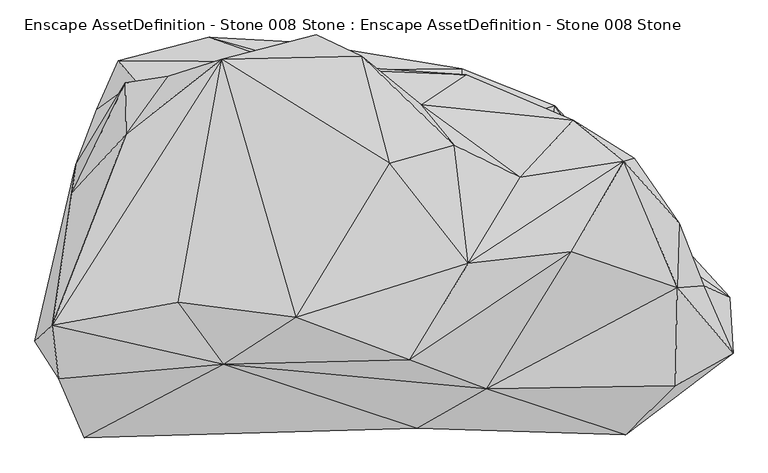
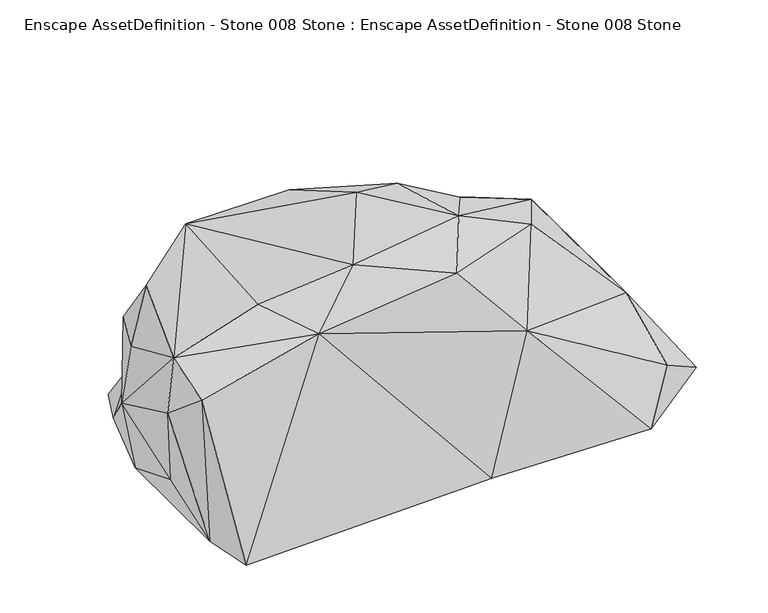
"""IFC4 building model written with IfcOpenShell, lengths in millimetres: geographic element geometry, Enscape AssetDefinition - Stone 008 Stone : Enscape AssetDefinition - Stone 008 Stone."""

import ifcopenshell
import ifcopenshell.guid

model = None  # the IFC model being written
_history = None  # IfcOwnerHistory: only IFC2X3 demands one
_inside = {}  # id of a spatial element -> (the spatial element, [elements in it])
_under = {}  # id of a project, library or spatial element -> (it, [spatial elements below it])
_declared = {}  # id of a project -> (the project, [libraries it declares])
_typed = {}  # id of a type object -> (the type object, [elements of that type])
_made_of = {}  # id of a material, layer set ... -> (it, [elements and type objects made of it])


def new_model(schema):
    """Start an empty IFC model of exactly this schema.

    Asked for "IFC4X3", IfcOpenShell would pick the latest addendum, in which some entities
    have other attributes; the version numbers below select the first issue.
    IFC2X3 requires an IfcOwnerHistory on every rooted entity: one is made here for all.
    """
    global model, _history
    if schema == "IFC4X3":
        model = ifcopenshell.file(schema_version=(4, 3, 0, 0))
    else:
        model = ifcopenshell.file(schema=schema)
    _inside.clear()
    _under.clear()
    _declared.clear()
    _typed.clear()
    _made_of.clear()
    _history = None
    if model.schema == "IFC2X3":
        org = make("IfcOrganization", Name="unknown")
        user = make(
            "IfcPersonAndOrganization",
            ThePerson=make("IfcPerson", FamilyName="unknown"),
            TheOrganization=org,
        )
        app = make(
            "IfcApplication",
            ApplicationDeveloper=org,
            Version="unknown",
            ApplicationFullName="unknown",
            ApplicationIdentifier="unknown",
        )
        _history = make(
            "IfcOwnerHistory",
            OwningUser=user,
            OwningApplication=app,
            ChangeAction="ADDED",
            CreationDate=0,
        )
    return model


def make(cls, **values):
    """One entity of the class cls with the attributes given. An attribute that is None is left unset."""
    return model.create_entity(
        cls, **{name: value for name, value in values.items() if value is not None}
    )


def rooted(cls, **values):
    """An entity with a GlobalId (a new one), such as an element, a storey or a relation."""
    return make(cls, GlobalId=ifcopenshell.guid.new(), OwnerHistory=_history, **values)


def si_unit(unit_type, name, prefix=None):
    """IfcSIUnit, for example si_unit("LENGTHUNIT", "METRE", prefix="MILLI")."""
    return make("IfcSIUnit", UnitType=unit_type, Prefix=prefix, Name=name)


def assignment(units):
    """IfcUnitAssignment: the units of a project."""
    return None if units is None else make("IfcUnitAssignment", Units=units)


def point(xyz):
    """IfcCartesianPoint."""
    return None if xyz is None else make("IfcCartesianPoint", Coordinates=xyz)


def direction(xyz):
    """IfcDirection."""
    return None if xyz is None else make("IfcDirection", DirectionRatios=xyz)


def frame(location, z_axis=None, x_axis=None):
    """IfcAxis2Placement3D, a coordinate frame: its origin and axes. An axis left out is left unset."""
    return make(
        "IfcAxis2Placement3D",
        Location=point(location),
        Axis=direction(z_axis),
        RefDirection=direction(x_axis),
    )


def origin():
    """The frame at (0, 0, 0) with its axes left unset."""
    return frame((0.0, 0.0, 0.0))


def place(relative_to, where):
    """IfcLocalPlacement: puts the frame where relative to a parent placement (None: the world)."""
    return make(
        "IfcLocalPlacement", PlacementRelTo=relative_to, RelativePlacement=where
    )


def context(
    kind, dimensions, precision=None, world=None, true_north=None, identifier=None
):
    """IfcGeometricRepresentationContext, for example the 3D "Model" context."""
    return make(
        "IfcGeometricRepresentationContext",
        ContextIdentifier=identifier,
        ContextType=kind,
        CoordinateSpaceDimension=dimensions,
        Precision=precision,
        WorldCoordinateSystem=world,
        TrueNorth=true_north,
    )


def project(units=None, contexts=None):
    """IfcProject with its units and contexts."""
    return rooted(
        "IfcProject",
        Name="project",
        RepresentationContexts=contexts,
        UnitsInContext=assignment(units),
    )


def spatial(cls, under=None, at=None, **own):
    """A site, building, storey or space (cls), placed at a placement, below another one or the project."""
    s = rooted(cls, ObjectPlacement=at, **own)
    if under is not None:
        _under.setdefault(under.id(), (under, []))[1].append(s)
    return s


def faces_of(points, faces, orient=None, outer=None):
    """IfcFace entities. A face is a list of loops; a loop is a list of indices into points, from 0.

    orient and outer hold one flag for each loop. By default every Orientation is true, the
    first loop of a face is its IfcFaceOuterBound and the others are IfcFaceBound.
    """
    made = []
    for i, loops in enumerate(faces):
        bounds = []
        for j, loop in enumerate(loops):
            is_outer = j == 0 if outer is None else outer[i][j]
            bounds.append(
                make(
                    "IfcFaceOuterBound" if is_outer else "IfcFaceBound",
                    Bound=make("IfcPolyLoop", Polygon=[points[k] for k in loop]),
                    Orientation=True if orient is None else orient[i][j],
                )
            )
        made.append(make("IfcFace", Bounds=bounds))
    return made


def faceted_brep(points, faces, orient=None, outer=None, voids=None):
    """IfcFacetedBrep: a solid bounded by flat faces; with voids (closed shells), ...WithVoids."""
    shared = [point(p) for p in points]
    hull = make("IfcClosedShell", CfsFaces=faces_of(shared, faces, orient, outer))
    if voids is None:
        return make("IfcFacetedBrep", Outer=hull)
    return make(
        "IfcFacetedBrepWithVoids",
        Outer=hull,
        Voids=[
            make(cls, CfsFaces=faces_of(shared, fs, o, b)) for cls, fs, o, b in voids
        ],
    )


def shape(context_of_items, identifier, shape_type, items):
    """IfcShapeRepresentation: the items that make up one representation, for example the "Body"."""
    return make(
        "IfcShapeRepresentation",
        ContextOfItems=context_of_items,
        RepresentationIdentifier=identifier,
        RepresentationType=shape_type,
        Items=items,
    )


def source(mapping_origin, context_of_items, identifier, shape_type, items):
    """IfcRepresentationMap: a shape defined once, which mapped items show again and again."""
    return make(
        "IfcRepresentationMap",
        MappingOrigin=mapping_origin,
        MappedRepresentation=shape(context_of_items, identifier, shape_type, items),
    )


def transform(
    local_origin,
    x_axis=None,
    y_axis=None,
    z_axis=None,
    scale=None,
    scale2=None,
    scale3=None,
    uniform=True,
):
    """IfcCartesianTransformationOperator3D, or its non-uniform kind. x_axis, y_axis, z_axis: its Axis1, 2, 3."""
    if uniform:
        return make(
            "IfcCartesianTransformationOperator3D",
            Axis1=direction(x_axis),
            Axis2=direction(y_axis),
            LocalOrigin=point(local_origin),
            Scale=scale,
            Axis3=direction(z_axis),
        )
    return make(
        "IfcCartesianTransformationOperator3DnonUniform",
        Axis1=direction(x_axis),
        Axis2=direction(y_axis),
        LocalOrigin=point(local_origin),
        Scale=scale,
        Axis3=direction(z_axis),
        Scale2=scale2,
        Scale3=scale3,
    )


def mapped(mapping_source, mapping_target):
    """IfcMappedItem: shows the shape of a source again, moved by a transform."""
    return make(
        "IfcMappedItem", MappingSource=mapping_source, MappingTarget=mapping_target
    )


def made_of(thing, what):
    """Note that an element or type object is made of a material, layer set ...; save() writes the relation."""
    if what is not None:
        _made_of.setdefault(what.id(), (what, []))[1].append(thing)
    return thing


def element(
    cls,
    number,
    at=None,
    inside=None,
    cuts=None,
    type_object=None,
    material=None,
    context=None,
    identifier="Body",
    shape_type=None,
    held_by="IfcProductDefinitionShape",
    body=None,
    shapes=None,
    **own,
):
    """One element of the class cls, such as IfcWall. Its Tag is "e" and its number.

    at: its placement. inside: the storey or other place that contains it. cuts: it is an
    opening in that element (IfcRelVoidsElement). A single representation is given by context,
    identifier, shape_type and body (its items); several are given by shapes. held_by: the class
    of the entity that holds the representations. save() writes the other relations.
    """
    e = rooted(cls, Tag="e%d" % number, ObjectPlacement=at, **own)
    if body is not None:
        shapes = [shape(context, identifier, shape_type, body)]
    if shapes is not None:
        e.Representation = make(held_by, Representations=shapes)
    if inside is not None:
        _inside.setdefault(inside.id(), (inside, []))[1].append(e)
    if cuts is not None:
        rooted(
            "IfcRelVoidsElement", RelatingBuildingElement=cuts, RelatedOpeningElement=e
        )
    if type_object is not None:
        _typed.setdefault(type_object.id(), (type_object, []))[1].append(e)
    return made_of(e, material)


def aggregate(whole, parts):
    """IfcRelAggregates: a whole, such as a stair, and the parts it consists of."""
    return rooted("IfcRelAggregates", RelatingObject=whole, RelatedObjects=parts)


def save(model, path):
    """Write the relations noted so far, then the file.

    IfcRelAggregates (storeys below a building ...), IfcRelContainedInSpatialStructure (elements
    in a storey), IfcRelDefinesByType, IfcRelAssociatesMaterial and IfcRelDeclares: one each for
    every whole, place, type object, material and project.
    """
    for whole, parts in _under.values():
        aggregate(whole, parts)
    for where, things in _inside.values():
        rooted(
            "IfcRelContainedInSpatialStructure",
            RelatedElements=things,
            RelatingStructure=where,
        )
    for kind, things in _typed.values():
        rooted("IfcRelDefinesByType", RelatedObjects=things, RelatingType=kind)
    for what, things in _made_of.values():
        rooted("IfcRelAssociatesMaterial", RelatedObjects=things, RelatingMaterial=what)
    for by, libraries in _declared.values():
        rooted("IfcRelDeclares", RelatingContext=by, RelatedDefinitions=libraries)
    model.write(path)


def enscape_assetdefinition_stone_008_stone_enscape_24533d0f(model_context):
    return source(origin(), model_context, "Body", "Brep", [
        faceted_brep([(674.4772792, 188.1209314, 142.7758336), (1035.7327461, 8.9201359, 108.4343269), (705.4293752, 497.0492125, 9.8005356), (997.1603155, 302.5434315, 403.4194052), (1162.8789902, 63.3667782, 307.4120581), (1253.1027794, -166.4617509, 132.1936697), (1349.0210772, -208.1131637, 6.9734799), (358.8430882, 390.0140226, 146.3160366), (377.8702021, 610.8905673, 436.6148412), (958.5034251, 293.037504, 588.9674425), (772.0807195, 443.9393878, 571.6524124), (1155.1955938, -174.3785888, 316.583544), (1361.7579937, -414.6891236, 4.4628736), (966.4069414, -714.6763802, 5.4843184), (1148.0065584, -535.101831, 161.3812745), (454.9190998, -545.4375148, 589.6245837), (765.6313181, -41.1196649, 728.256464), (197.4091679, -690.6881928, 2.2398918), (-514.082849, -456.0222328, 858.2776785), (170.5874205, -438.8919473, 922.1434593), (385.2636814, -83.5196525, 931.4427376), (-247.4171519, -282.6159894, 1018.4793472), (576.8572688, 233.5522175, 768.9470053), (335.1638615, 351.0840833, 853.2254696), (97.4461734, 284.5808566, 931.3715696), (213.0276859, 499.7121692, 607.2036028), (-6.4782458, 678.3997416, 740.2927279), (-523.0283737, 667.5286889, 753.1849146), (-682.7530861, -228.3637375, 932.9548478), (-874.7516274, 392.5074339, 724.0793109), (-1147.2679377, -313.0920827, 869.5514202), (-173.4227836, 757.5678229, 583.3979845), (-719.4939852, 606.0778499, 573.5012889), (-121.4118823, 631.9727302, 438.7468398), (-477.7078629, 640.0285363, 443.1231916), (-877.9751062, 580.4912448, 445.3162253), (-1074.303627, 173.3499914, 609.6158624), (-1061.0442162, 279.8386514, 242.5745577), (-839.9647474, 586.9014859, 173.4158546), (-312.4943078, 658.5144997, 220.8529711), (-903.9554596, 662.9179716, 4.3747872), (-983.217001, 483.1243753, 17.7407339), (-570.9864497, 749.253273, 0.3116064), (-136.2574697, 627.3009181, 146.1777389), (-233.8543534, 731.0650349, 7.1665621), (362.7277911, 632.3495507, 5.9714052), (-1086.7136717, 120.3676835, 13.3715561), (-1058.6297512, -132.5317025, 94.683297), (-1091.7432308, -525.1657367, 26.3983011), (-1029.1792154, -726.3221741, 1.9205989), (-1210.739255, -371.0243106, 639.5069957), (-1122.2990751, -508.4093809, 759.0334415)], [[[0, 1, 2]], [[3, 4, 1]], [[4, 5, 1]], [[1, 5, 6]], [[3, 1, 0]], [[2, 1, 6]], [[0, 2, 7]], [[7, 8, 0]], [[0, 8, 3]], [[3, 9, 4]], [[10, 3, 8]], [[3, 10, 9]], [[9, 11, 4]], [[4, 11, 5]], [[12, 5, 11]], [[12, 6, 5]], [[13, 2, 6]], [[13, 6, 12]], [[12, 11, 14]], [[12, 14, 13]], [[11, 15, 14]], [[16, 15, 11]], [[11, 9, 16]], [[14, 15, 13]], [[13, 15, 17]], [[13, 17, 2]], [[18, 15, 19]], [[16, 19, 15]], [[18, 17, 15]], [[16, 20, 19]], [[16, 9, 20]], [[21, 19, 20]], [[21, 18, 19]], [[9, 22, 20]], [[20, 22, 23]], [[20, 23, 24]], [[24, 21, 20]], [[10, 22, 9]], [[23, 22, 25]], [[25, 22, 10]], [[23, 26, 24]], [[25, 26, 23]], [[27, 21, 24]], [[27, 24, 26]], [[27, 28, 21]], [[18, 21, 28]], [[27, 29, 30]], [[27, 26, 31]], [[31, 32, 27]], [[27, 30, 28]], [[27, 32, 29]], [[26, 25, 31]], [[31, 25, 33]], [[34, 32, 31]], [[33, 34, 31]], [[32, 34, 35]], [[32, 35, 29]], [[29, 36, 30]], [[29, 35, 36]], [[35, 37, 36]], [[38, 37, 35]], [[38, 35, 34]], [[38, 34, 33]], [[25, 8, 33]], [[39, 38, 33]], [[8, 39, 33]], [[38, 40, 41]], [[37, 38, 41]], [[39, 40, 38]], [[39, 42, 40]], [[8, 43, 39]], [[42, 39, 43]], [[10, 8, 25]], [[43, 8, 7]], [[44, 43, 45]], [[44, 42, 43]], [[45, 43, 7]], [[42, 46, 41]], [[42, 41, 40]], [[46, 42, 44]], [[41, 46, 37]], [[47, 46, 48]], [[47, 37, 46]], [[46, 44, 17]], [[17, 48, 46]], [[17, 44, 45]], [[7, 2, 45]], [[17, 45, 2]], [[48, 17, 49]], [[18, 49, 17]], [[50, 48, 51]], [[47, 48, 50]], [[51, 48, 49]], [[37, 47, 50]], [[50, 51, 30]], [[50, 30, 37]], [[36, 37, 30]], [[18, 28, 30]], [[51, 18, 30]], [[49, 18, 51]]]),
    ])


if __name__ == "__main__":
    model = new_model("IFC4")
    model_context = context("Model", 3, world=origin())
    ifc_project = project(units=[si_unit("LENGTHUNIT", "METRE", prefix="MILLI")], contexts=[model_context])
    site = spatial("IfcSite", under=ifc_project)
    building = spatial("IfcBuilding", under=site)
    placement = place(None, origin())
    enscape_assetdefinition_stone_008_stone_enscape_shape = enscape_assetdefinition_stone_008_stone_enscape_24533d0f(model_context)
    element("IfcGeographicElement", 1, ObjectType="Enscape AssetDefinition - Stone 008 Stone : Enscape AssetDefinition - Stone 008 Stone", at=placement, inside=building, context=model_context, shape_type="MappedRepresentation", body=[
        mapped(enscape_assetdefinition_stone_008_stone_enscape_shape, transform((0.0, 0.0, 0.0), x_axis=(1.0, 0.0, 0.0), y_axis=(0.0, 1.0, 0.0), z_axis=(0.0, 0.0, 1.0))),
    ])
    save(model, "model.ifc")

# Revit data of these elements
# Type "Enscape AssetDefinition - Stone 008 Stone : Enscape AssetDefinition - Stone 008 Stone"
#   EnscapeAssetSource = "REMOTE"
#   EnscapeAssetId = "21c0a78a-166e-4c5c-8e35-d18d7a930555"
#   Height = 1.018479 m
#   EnscapeNativeAssetHeight = 1.018479 m
#   Default Elevation = 0
